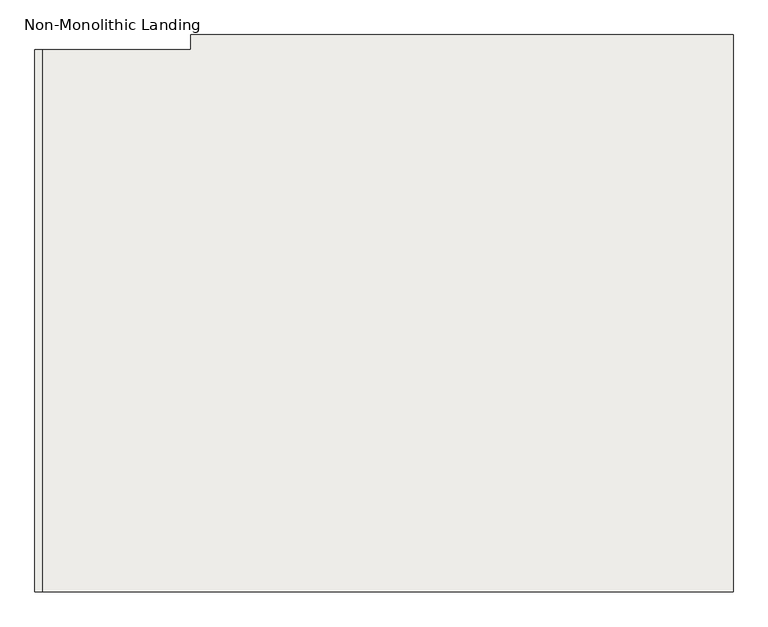
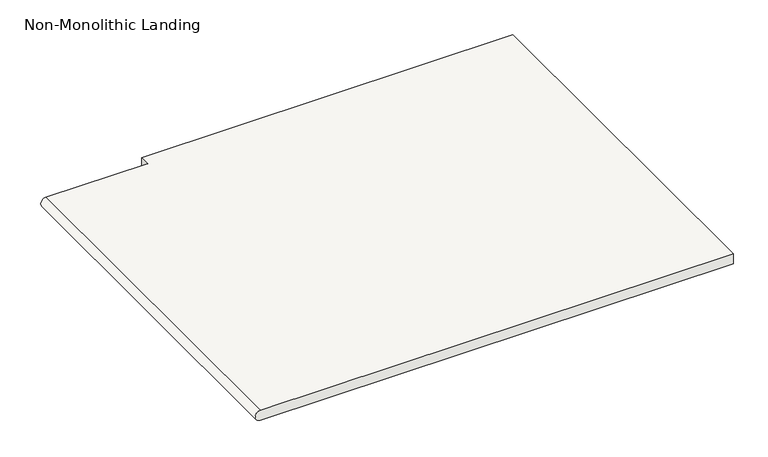
"""IFC4 building model written with IfcOpenShell, lengths in millimetres: slab geometry, Non-Monolithic Landing."""

import ifcopenshell
import ifcopenshell.guid

model = None  # the IFC model being written
_history = None  # IfcOwnerHistory: only IFC2X3 demands one
_inside = {}  # id of a spatial element -> (the spatial element, [elements in it])
_under = {}  # id of a project, library or spatial element -> (it, [spatial elements below it])
_declared = {}  # id of a project -> (the project, [libraries it declares])
_typed = {}  # id of a type object -> (the type object, [elements of that type])
_made_of = {}  # id of a material, layer set ... -> (it, [elements and type objects made of it])


def new_model(schema):
    """Start an empty IFC model of exactly this schema.

    Asked for "IFC4X3", IfcOpenShell would pick the latest addendum, in which some entities
    have other attributes; the version numbers below select the first issue.
    IFC2X3 requires an IfcOwnerHistory on every rooted entity: one is made here for all.
    """
    global model, _history
    if schema == "IFC4X3":
        model = ifcopenshell.file(schema_version=(4, 3, 0, 0))
    else:
        model = ifcopenshell.file(schema=schema)
    _inside.clear()
    _under.clear()
    _declared.clear()
    _typed.clear()
    _made_of.clear()
    _history = None
    if model.schema == "IFC2X3":
        org = make("IfcOrganization", Name="unknown")
        user = make(
            "IfcPersonAndOrganization",
            ThePerson=make("IfcPerson", FamilyName="unknown"),
            TheOrganization=org,
        )
        app = make(
            "IfcApplication",
            ApplicationDeveloper=org,
            Version="unknown",
            ApplicationFullName="unknown",
            ApplicationIdentifier="unknown",
        )
        _history = make(
            "IfcOwnerHistory",
            OwningUser=user,
            OwningApplication=app,
            ChangeAction="ADDED",
            CreationDate=0,
        )
    return model


def make(cls, **values):
    """One entity of the class cls with the attributes given. An attribute that is None is left unset."""
    return model.create_entity(
        cls, **{name: value for name, value in values.items() if value is not None}
    )


def rooted(cls, **values):
    """An entity with a GlobalId (a new one), such as an element, a storey or a relation."""
    return make(cls, GlobalId=ifcopenshell.guid.new(), OwnerHistory=_history, **values)


def si_unit(unit_type, name, prefix=None):
    """IfcSIUnit, for example si_unit("LENGTHUNIT", "METRE", prefix="MILLI")."""
    return make("IfcSIUnit", UnitType=unit_type, Prefix=prefix, Name=name)


def assignment(units):
    """IfcUnitAssignment: the units of a project."""
    return None if units is None else make("IfcUnitAssignment", Units=units)


def point(xyz):
    """IfcCartesianPoint."""
    return None if xyz is None else make("IfcCartesianPoint", Coordinates=xyz)


def direction(xyz):
    """IfcDirection."""
    return None if xyz is None else make("IfcDirection", DirectionRatios=xyz)


def frame(location, z_axis=None, x_axis=None):
    """IfcAxis2Placement3D, a coordinate frame: its origin and axes. An axis left out is left unset."""
    return make(
        "IfcAxis2Placement3D",
        Location=point(location),
        Axis=direction(z_axis),
        RefDirection=direction(x_axis),
    )


def origin():
    """The frame at (0, 0, 0) with its axes left unset."""
    return frame((0.0, 0.0, 0.0))


def place(relative_to, where):
    """IfcLocalPlacement: puts the frame where relative to a parent placement (None: the world)."""
    return make(
        "IfcLocalPlacement", PlacementRelTo=relative_to, RelativePlacement=where
    )


def context(
    kind, dimensions, precision=None, world=None, true_north=None, identifier=None
):
    """IfcGeometricRepresentationContext, for example the 3D "Model" context."""
    return make(
        "IfcGeometricRepresentationContext",
        ContextIdentifier=identifier,
        ContextType=kind,
        CoordinateSpaceDimension=dimensions,
        Precision=precision,
        WorldCoordinateSystem=world,
        TrueNorth=true_north,
    )


def project(units=None, contexts=None):
    """IfcProject with its units and contexts."""
    return rooted(
        "IfcProject",
        Name="project",
        RepresentationContexts=contexts,
        UnitsInContext=assignment(units),
    )


def spatial(cls, under=None, at=None, **own):
    """A site, building, storey or space (cls), placed at a placement, below another one or the project."""
    s = rooted(cls, ObjectPlacement=at, **own)
    if under is not None:
        _under.setdefault(under.id(), (under, []))[1].append(s)
    return s


def circle_curve(where, radius):
    """IfcCircle in the frame where."""
    return make("IfcCircle", Position=where, Radius=radius)


def shape(context_of_items, identifier, shape_type, items):
    """IfcShapeRepresentation: the items that make up one representation, for example the "Body"."""
    return make(
        "IfcShapeRepresentation",
        ContextOfItems=context_of_items,
        RepresentationIdentifier=identifier,
        RepresentationType=shape_type,
        Items=items,
    )


def source(mapping_origin, context_of_items, identifier, shape_type, items):
    """IfcRepresentationMap: a shape defined once, which mapped items show again and again."""
    return make(
        "IfcRepresentationMap",
        MappingOrigin=mapping_origin,
        MappedRepresentation=shape(context_of_items, identifier, shape_type, items),
    )


def transform(
    local_origin,
    x_axis=None,
    y_axis=None,
    z_axis=None,
    scale=None,
    scale2=None,
    scale3=None,
    uniform=True,
):
    """IfcCartesianTransformationOperator3D, or its non-uniform kind. x_axis, y_axis, z_axis: its Axis1, 2, 3."""
    if uniform:
        return make(
            "IfcCartesianTransformationOperator3D",
            Axis1=direction(x_axis),
            Axis2=direction(y_axis),
            LocalOrigin=point(local_origin),
            Scale=scale,
            Axis3=direction(z_axis),
        )
    return make(
        "IfcCartesianTransformationOperator3DnonUniform",
        Axis1=direction(x_axis),
        Axis2=direction(y_axis),
        LocalOrigin=point(local_origin),
        Scale=scale,
        Axis3=direction(z_axis),
        Scale2=scale2,
        Scale3=scale3,
    )


def mapped(mapping_source, mapping_target):
    """IfcMappedItem: shows the shape of a source again, moved by a transform."""
    return make(
        "IfcMappedItem", MappingSource=mapping_source, MappingTarget=mapping_target
    )


def made_of(thing, what):
    """Note that an element or type object is made of a material, layer set ...; save() writes the relation."""
    if what is not None:
        _made_of.setdefault(what.id(), (what, []))[1].append(thing)
    return thing


def element(
    cls,
    number,
    at=None,
    inside=None,
    cuts=None,
    type_object=None,
    material=None,
    context=None,
    identifier="Body",
    shape_type=None,
    held_by="IfcProductDefinitionShape",
    body=None,
    shapes=None,
    **own,
):
    """One element of the class cls, such as IfcWall. Its Tag is "e" and its number.

    at: its placement. inside: the storey or other place that contains it. cuts: it is an
    opening in that element (IfcRelVoidsElement). A single representation is given by context,
    identifier, shape_type and body (its items); several are given by shapes. held_by: the class
    of the entity that holds the representations. save() writes the other relations.
    """
    e = rooted(cls, Tag="e%d" % number, ObjectPlacement=at, **own)
    if body is not None:
        shapes = [shape(context, identifier, shape_type, body)]
    if shapes is not None:
        e.Representation = make(held_by, Representations=shapes)
    if inside is not None:
        _inside.setdefault(inside.id(), (inside, []))[1].append(e)
    if cuts is not None:
        rooted(
            "IfcRelVoidsElement", RelatingBuildingElement=cuts, RelatedOpeningElement=e
        )
    if type_object is not None:
        _typed.setdefault(type_object.id(), (type_object, []))[1].append(e)
    return made_of(e, material)


def aggregate(whole, parts):
    """IfcRelAggregates: a whole, such as a stair, and the parts it consists of."""
    return rooted("IfcRelAggregates", RelatingObject=whole, RelatedObjects=parts)


def save(model, path):
    """Write the relations noted so far, then the file.

    IfcRelAggregates (storeys below a building ...), IfcRelContainedInSpatialStructure (elements
    in a storey), IfcRelDefinesByType, IfcRelAssociatesMaterial and IfcRelDeclares: one each for
    every whole, place, type object, material and project.
    """
    for whole, parts in _under.values():
        aggregate(whole, parts)
    for where, things in _inside.values():
        rooted(
            "IfcRelContainedInSpatialStructure",
            RelatedElements=things,
            RelatingStructure=where,
        )
    for kind, things in _typed.values():
        rooted("IfcRelDefinesByType", RelatedObjects=things, RelatingType=kind)
    for what, things in _made_of.values():
        rooted("IfcRelAssociatesMaterial", RelatedObjects=things, RelatingMaterial=what)
    for by, libraries in _declared.values():
        rooted("IfcRelDeclares", RelatingContext=by, RelatedDefinitions=libraries)
    model.write(path)


def plane_surface(at):
    """IfcPlane: the flat surface through the origin of the frame at, square to its z axis."""
    return make("IfcPlane", Position=at)


def cylinder_surface(at, radius):
    """IfcCylindricalSurface: all points at the distance radius from the z axis of the frame at."""
    return make("IfcCylindricalSurface", Position=at, Radius=radius)


def advanced_brep(points, edges, surfaces, faces):
    """IfcAdvancedBrep: a solid bounded by faces that lie on surfaces and meet in shared edges.

    An edge is (start, end): straight between two places in points (the first is 0);
    or (start, end, curve); or (start, end, curve, False) where it runs against its curve.
    A face is (place in surfaces, loops), or (place, loops, False) where it looks against
    its surface's normal. A loop lists edges by number (the first is 1), with a minus sign
    where the edge is run from its end to its start. The first loop is the outer one.
    """
    corners = [point(p) for p in points]
    vertices = [make("IfcVertexPoint", VertexGeometry=c) for c in corners]
    made = []
    for start, end, *more in edges:
        made.append(
            make(
                "IfcEdgeCurve",
                EdgeStart=vertices[start],
                EdgeEnd=vertices[end],
                EdgeGeometry=more[0] if more else make("IfcPolyline", Points=[corners[start], corners[end]]),
                SameSense=more[1] if len(more) > 1 else True,
            )
        )
    hull = []
    for where, loops, *sense in faces:
        bounds = []
        for j, loop in enumerate(loops):
            ring = [make("IfcOrientedEdge", EdgeElement=made[abs(k) - 1], Orientation=k > 0) for k in loop]
            bounds.append(
                make(
                    "IfcFaceOuterBound" if j == 0 else "IfcFaceBound",
                    Bound=make("IfcEdgeLoop", EdgeList=ring),
                    Orientation=True,
                )
            )
        hull.append(make("IfcAdvancedFace", Bounds=bounds, FaceSurface=surfaces[where], SameSense=sense[0] if sense else True))
    return make("IfcAdvancedBrep", Outer=make("IfcClosedShell", CfsFaces=hull))


def non_monolithic_landing_e3905461(model_context):
    return source(origin(), model_context, "Body", "AdvancedBrep", [
        advanced_brep(
        [(6239.7741968, -13363.3557429, 4432.3), (6239.7741968, -13363.3557429, 4457.7), (6239.7741968, -12448.9557429, 4457.7), (6239.7741968, -12448.9557429, 4432.3), (7404.2789345, -13363.3557429, 4457.7), (7404.2789345, -12448.9557429, 4457.7), (7404.2789345, -12423.5557429, 4457.7), (6489.8789345, -12423.5557429, 4457.7), (6489.8789345, -12448.9557429, 4457.7), (7404.2789345, -13363.3557429, 4432.3), (6489.8789345, -12448.9557429, 4432.3), (6489.8789345, -12423.5557429, 4432.3), (7404.2789345, -12423.5557429, 4432.3), (7404.2789345, -12448.9557429, 4432.3)],
        [
            (0, 1, circle_curve(frame((6239.7741968, -13363.3557429, 4445.0), z_axis=(0.0, 1.0, 0.0), x_axis=(1.0, 0.0, 0.0)), 12.7)),
            (1, 2),
            (2, 3, circle_curve(frame((6239.7741968, -12448.9557429, 4445.0), z_axis=(0.0, -1.0, 0.0), x_axis=(1.0, 0.0, 0.0)), 12.7)),
            (3, 0),
            (1, 4),
            (4, 5),
            (5, 6),
            (6, 7),
            (7, 8),
            (8, 2),
            (9, 0),
            (3, 10),
            (10, 11),
            (11, 12),
            (12, 13),
            (13, 9),
            (9, 4),
            (13, 5),
            (12, 6),
            (11, 7),
            (10, 8),
        ],
        [
            cylinder_surface(frame((6239.7741968, -13363.3557429, 4445.0), z_axis=(0.0, -1.0, 0.0), x_axis=(1.0, 0.0, 0.0)), 12.7),
            plane_surface(frame((6239.7741968, -12448.9557429, 4457.7), z_axis=(0.0, 0.0, 1.0), x_axis=(0.0, -1.0, 0.0))),
            plane_surface(frame((6239.7741968, -12448.9557429, 4432.3), z_axis=(0.0, 0.0, -1.0), x_axis=(0.0, 1.0, 0.0))),
            plane_surface(frame((6239.7741968, -13363.3557429, 4457.7), z_axis=(0.0, -1.0, 0.0), x_axis=(0.0, 0.0, -1.0))),
            plane_surface(frame((7404.2789345, -13363.3557429, 4457.7), z_axis=(1.0, 0.0, 0.0), x_axis=(0.0, 0.0, -1.0))),
            plane_surface(frame((7404.2789345, -12448.9557429, 4457.7), z_axis=(1.0, 0.0, 0.0), x_axis=(0.0, 0.0, -1.0))),
            plane_surface(frame((7404.2789345, -12423.5557429, 4457.7), z_axis=(0.0, 1.0, 0.0), x_axis=(0.0, 0.0, -1.0))),
            plane_surface(frame((6489.8789345, -12423.5557429, 4457.7), z_axis=(-1.0, 0.0, 0.0), x_axis=(0.0, 0.0, -1.0))),
            plane_surface(frame((6489.8789345, -12448.9557429, 4457.7), z_axis=(0.0, 1.0, 0.0), x_axis=(0.0, 0.0, -1.0))),
        ],
        [
            (0, [[1, 2, 3, 4]]),
            (1, [[5, 6, 7, 8, 9, 10, -2]]),
            (2, [[11, -4, 12, 13, 14, 15, 16]]),
            (3, [[-5, -1, -11, 17]]),
            (4, [[-6, -17, -16, 18]]),
            (5, [[-7, -18, -15, 19]]),
            (6, [[-8, -19, -14, 20]]),
            (7, [[-9, -20, -13, 21]]),
            (8, [[-10, -21, -12, -3]]),
        ],
    ),
    ])


if __name__ == "__main__":
    model = new_model("IFC4")
    model_context = context("Model", 3, world=origin())
    ifc_project = project(units=[si_unit("LENGTHUNIT", "METRE", prefix="MILLI")], contexts=[model_context])
    site = spatial("IfcSite", under=ifc_project)
    building = spatial("IfcBuilding", under=site)
    placement = place(None, origin())
    non_monolithic_landing_shape = non_monolithic_landing_e3905461(model_context)
    element("IfcSlab", 1, ObjectType="Non-Monolithic Landing", at=placement, inside=building, context=model_context, shape_type="MappedRepresentation", body=[
        mapped(non_monolithic_landing_shape, transform((0.0, 0.0, 0.0), x_axis=(1.0, 0.0, 0.0), y_axis=(0.0, 1.0, 0.0), z_axis=(0.0, 0.0, 1.0))),
    ])
    save(model, "model.ifc")

# Revit data of these elements
# Element 1 (IfcSlab, "Non-Monolithic Landing")
#   Materials on its faces: "Cherry"
# Materials
#   "Cherry": class "Wood", colour RGB 233 182 144, transparency 0, Description = "Prunus Serotina", Cost = 0
